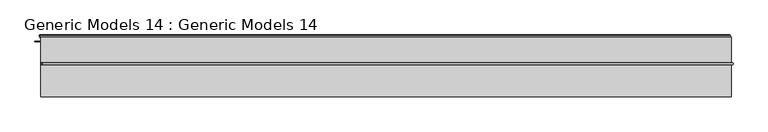
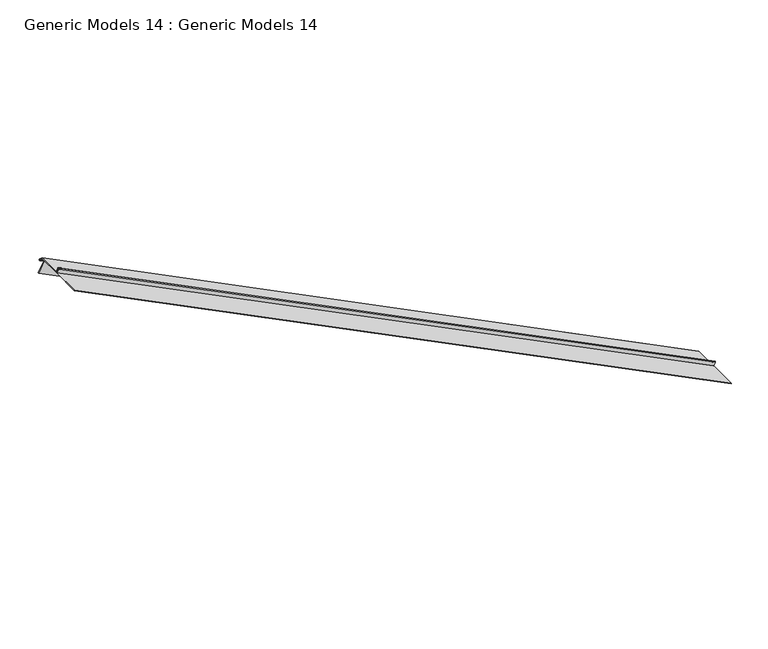
"""IFC4 building model written with IfcOpenShell, lengths in millimetres: proxy geometry, Generic Models 14 : Generic Models 14."""

from ifc_helpers import new_model, si_unit, point, frame, frame_2d, origin, place, context, project, spatial, polyline, circle_curve, trimmed, segment, composite_curve, outline, extrude, source, transform, mapped, element, save


def generic_models_14_generic_models_14_81b2d5b4(model_context):
    return source(origin(), model_context, "Body", "SweptSolid", [
        extrude(outline(composite_curve([segment(polyline([(29.765625, 0.0), (43.2360092, 13.4703842)]), True, "CONTINUOUS"), segment(trimmed(circle_curve(frame_2d((41.148799, 15.5575944)), 2.951761), [point((43.2360092, 13.4703842))], [point((39.0615888, 17.6448046))], True, "CARTESIAN"), True, "CONTINUOUS"), segment(polyline([(39.0615888, 17.6448046), (27.5755796, 6.1587955), (26.4530476, 7.2813274), (37.9390568, 18.7673366)]), True, "CONTINUOUS"), segment(trimmed(circle_curve(frame_2d((41.148799, 15.5575944)), 4.539261), [point((37.9390568, 18.7673366))], [point((44.3585412, 12.3478522))], False, "CARTESIAN"), True, "CONTINUOUS"), segment(polyline([(44.3585412, 12.3478522), (30.423189, -1.5875), (-130.0884673, -1.5875), (-130.0884673, -21.9670716)]), True, "CONTINUOUS"), segment(trimmed(circle_curve(frame_2d((-128.8525457, -21.9670716)), 1.2359216), [point((-130.0884673, -21.9670716))], [point((-127.616624, -21.9670716))], True, "CARTESIAN"), True, "CONTINUOUS"), segment(polyline([(-127.616624, -21.9670716), (-127.616624, -3.1749999), (-126.029124, -3.1749999), (-126.029124, -21.9670716)]), True, "CONTINUOUS"), segment(trimmed(circle_curve(frame_2d((-128.8525457, -21.9670716)), 2.8234216), [point((-126.029124, -21.9670716))], [point((-131.6759673, -21.9670716))], False, "CARTESIAN"), True, "CONTINUOUS"), segment(polyline([(-131.6759673, -21.9670716), (-131.6759673, 0.0), (29.765625, 0.0)]), True, "CONTINUOUS")], self_intersect=False)), frame((32077.6206029, 40951.6246078, 272265.91143), z_axis=(-0.8944271909999191, 0.0, 0.4472135954999516), x_axis=(0.0, 1.0, 0.0)), (0.0, 0.0, 1.0), 4676.5930666),
        extrude(outline(composite_curve([segment(polyline([(-125.3742498, -23.8213834), (-125.3742498, -5.0293119), (-123.7867498, -5.0293119), (-123.7867498, -23.8213834)]), True, "CONTINUOUS"), segment(trimmed(circle_curve(frame_2d((-128.9914215, -23.8213834)), 5.2046716), [point((-123.7867498, -23.8213834))], [point((-134.1960931, -23.8213834))], False, "CARTESIAN"), True, "CONTINUOUS"), segment(polyline([(-134.1960931, -23.8213834), (-134.1960931, -1.5875), (-328.7514466, -1.5875), (-328.7514466, 0.0), (-132.6085931, 0.0), (-132.6085931, -23.8213834)]), True, "CONTINUOUS"), segment(trimmed(circle_curve(frame_2d((-128.9914215, -23.8213834)), 3.6171716), [point((-132.6085931, -23.8213834))], [point((-125.3742498, -23.8213834))], True, "CARTESIAN"), True, "CONTINUOUS")], self_intersect=False)), frame((32077.6206029, 40951.6246078, 272265.91143), z_axis=(-0.8944271909999191, 0.0, 0.4472135954999516), x_axis=(0.0, 1.0, 0.0)), (0.0, 0.0, 1.0), 4676.5930666),
        extrude(outline(polyline([(0.0, 0.0), (0.0, -76.2000001), (21.7032521, -76.2000001), (34.3798862, -63.5233659), (35.5024182, -64.6458978), (22.3608161, -77.7875001), (-1.5875, -77.7875001), (-1.5875, 0.0), (0.0, 0.0)])), frame((32041.7680479, 40957.9746078, 272194.2063201), z_axis=(-0.8944271909999191, 0.0, 0.4472135954999516), x_axis=(-1.0365773547145834e-11, 1.0, -2.0737712226908407e-11)), (0.0, 0.0, 1.0), 4676.5930666),
    ])


if __name__ == "__main__":
    model = new_model("IFC4")
    model_context = context("Model", 3, world=origin())
    ifc_project = project(units=[si_unit("LENGTHUNIT", "METRE", prefix="MILLI")], contexts=[model_context])
    site = spatial("IfcSite", under=ifc_project)
    building = spatial("IfcBuilding", under=site)
    placement = place(None, origin())
    generic_models_14_generic_models_14_shape = generic_models_14_generic_models_14_81b2d5b4(model_context)
    element("IfcBuildingElementProxy", 1, Name="Generic Models 14 : Generic Models 14", ObjectType="Generic Models 14 : Generic Models 14", at=placement, inside=building, context=model_context, shape_type="MappedRepresentation", body=[
        mapped(generic_models_14_generic_models_14_shape, transform((0.0, 0.0, 0.0), x_axis=(1.0, 0.0, 0.0), y_axis=(0.0, 1.0, 0.0), z_axis=(0.0, 0.0, 1.0))),
    ])
    save(model, "model.ifc")

# Revit data of these elements
# Element 1 (IfcBuildingElementProxy, "Generic Models 14 : Generic Models 14")
#   Materials on its faces: "GALV. STANDING SEAM METAL ROOF", "GALV. BRAKE METAL - (COLOR: GALV.)"
# Materials
#   "GALV. STANDING SEAM METAL ROOF": class "Unassigned", colour RGB 228 228 228, transparency 0, Comments = "Rendering appearance not upgraded ", Description = "Standing Metal Seam Roof", Cost = 0
#   "GALV. BRAKE METAL - (COLOR: GALV.)": class "Generic", colour RGB 234 234 234, transparency 0, Cost = 0
